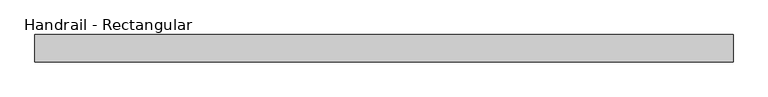
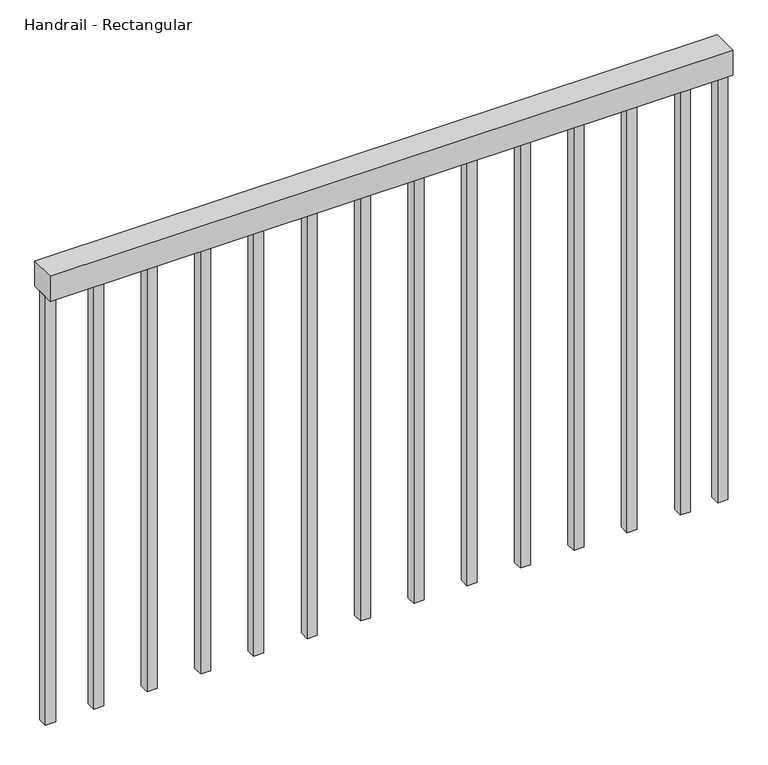
"""IFC4 building model written with IfcOpenShell, lengths in millimetres: railing geometry, Handrail - Rectangular."""

import ifcopenshell
import ifcopenshell.guid

model = None  # the IFC model being written
_history = None  # IfcOwnerHistory: only IFC2X3 demands one
_inside = {}  # id of a spatial element -> (the spatial element, [elements in it])
_under = {}  # id of a project, library or spatial element -> (it, [spatial elements below it])
_declared = {}  # id of a project -> (the project, [libraries it declares])
_typed = {}  # id of a type object -> (the type object, [elements of that type])
_made_of = {}  # id of a material, layer set ... -> (it, [elements and type objects made of it])


def new_model(schema):
    """Start an empty IFC model of exactly this schema.

    Asked for "IFC4X3", IfcOpenShell would pick the latest addendum, in which some entities
    have other attributes; the version numbers below select the first issue.
    IFC2X3 requires an IfcOwnerHistory on every rooted entity: one is made here for all.
    """
    global model, _history
    if schema == "IFC4X3":
        model = ifcopenshell.file(schema_version=(4, 3, 0, 0))
    else:
        model = ifcopenshell.file(schema=schema)
    _inside.clear()
    _under.clear()
    _declared.clear()
    _typed.clear()
    _made_of.clear()
    _history = None
    if model.schema == "IFC2X3":
        org = make("IfcOrganization", Name="unknown")
        user = make(
            "IfcPersonAndOrganization",
            ThePerson=make("IfcPerson", FamilyName="unknown"),
            TheOrganization=org,
        )
        app = make(
            "IfcApplication",
            ApplicationDeveloper=org,
            Version="unknown",
            ApplicationFullName="unknown",
            ApplicationIdentifier="unknown",
        )
        _history = make(
            "IfcOwnerHistory",
            OwningUser=user,
            OwningApplication=app,
            ChangeAction="ADDED",
            CreationDate=0,
        )
    return model


def make(cls, **values):
    """One entity of the class cls with the attributes given. An attribute that is None is left unset."""
    return model.create_entity(
        cls, **{name: value for name, value in values.items() if value is not None}
    )


def rooted(cls, **values):
    """An entity with a GlobalId (a new one), such as an element, a storey or a relation."""
    return make(cls, GlobalId=ifcopenshell.guid.new(), OwnerHistory=_history, **values)


def si_unit(unit_type, name, prefix=None):
    """IfcSIUnit, for example si_unit("LENGTHUNIT", "METRE", prefix="MILLI")."""
    return make("IfcSIUnit", UnitType=unit_type, Prefix=prefix, Name=name)


def assignment(units):
    """IfcUnitAssignment: the units of a project."""
    return None if units is None else make("IfcUnitAssignment", Units=units)


def point(xyz):
    """IfcCartesianPoint."""
    return None if xyz is None else make("IfcCartesianPoint", Coordinates=xyz)


def direction(xyz):
    """IfcDirection."""
    return None if xyz is None else make("IfcDirection", DirectionRatios=xyz)


def frame(location, z_axis=None, x_axis=None):
    """IfcAxis2Placement3D, a coordinate frame: its origin and axes. An axis left out is left unset."""
    return make(
        "IfcAxis2Placement3D",
        Location=point(location),
        Axis=direction(z_axis),
        RefDirection=direction(x_axis),
    )


def origin():
    """The frame at (0, 0, 0) with its axes left unset."""
    return frame((0.0, 0.0, 0.0))


def place(relative_to, where):
    """IfcLocalPlacement: puts the frame where relative to a parent placement (None: the world)."""
    return make(
        "IfcLocalPlacement", PlacementRelTo=relative_to, RelativePlacement=where
    )


def context(
    kind, dimensions, precision=None, world=None, true_north=None, identifier=None
):
    """IfcGeometricRepresentationContext, for example the 3D "Model" context."""
    return make(
        "IfcGeometricRepresentationContext",
        ContextIdentifier=identifier,
        ContextType=kind,
        CoordinateSpaceDimension=dimensions,
        Precision=precision,
        WorldCoordinateSystem=world,
        TrueNorth=true_north,
    )


def project(units=None, contexts=None):
    """IfcProject with its units and contexts."""
    return rooted(
        "IfcProject",
        Name="project",
        RepresentationContexts=contexts,
        UnitsInContext=assignment(units),
    )


def spatial(cls, under=None, at=None, **own):
    """A site, building, storey or space (cls), placed at a placement, below another one or the project."""
    s = rooted(cls, ObjectPlacement=at, **own)
    if under is not None:
        _under.setdefault(under.id(), (under, []))[1].append(s)
    return s


def polyline(points):
    """IfcPolyline through the points."""
    return make("IfcPolyline", Points=[point(p) for p in points])


def outline(outer, holes=None, kind="AREA"):
    """IfcArbitraryClosedProfileDef: a profile drawn as a closed curve; with holes, ...WithVoids."""
    if holes is None:
        return make("IfcArbitraryClosedProfileDef", ProfileType=kind, OuterCurve=outer)
    return make(
        "IfcArbitraryProfileDefWithVoids",
        ProfileType=kind,
        OuterCurve=outer,
        InnerCurves=holes,
    )


def extrude(swept, where, along, depth):
    """IfcExtrudedAreaSolid: the profile swept, set in the frame where, extruded along a direction by depth."""
    return make(
        "IfcExtrudedAreaSolid",
        SweptArea=swept,
        Position=where,
        ExtrudedDirection=direction(along),
        Depth=depth,
    )


def shape(context_of_items, identifier, shape_type, items):
    """IfcShapeRepresentation: the items that make up one representation, for example the "Body"."""
    return make(
        "IfcShapeRepresentation",
        ContextOfItems=context_of_items,
        RepresentationIdentifier=identifier,
        RepresentationType=shape_type,
        Items=items,
    )


def source(mapping_origin, context_of_items, identifier, shape_type, items):
    """IfcRepresentationMap: a shape defined once, which mapped items show again and again."""
    return make(
        "IfcRepresentationMap",
        MappingOrigin=mapping_origin,
        MappedRepresentation=shape(context_of_items, identifier, shape_type, items),
    )


def transform(
    local_origin,
    x_axis=None,
    y_axis=None,
    z_axis=None,
    scale=None,
    scale2=None,
    scale3=None,
    uniform=True,
):
    """IfcCartesianTransformationOperator3D, or its non-uniform kind. x_axis, y_axis, z_axis: its Axis1, 2, 3."""
    if uniform:
        return make(
            "IfcCartesianTransformationOperator3D",
            Axis1=direction(x_axis),
            Axis2=direction(y_axis),
            LocalOrigin=point(local_origin),
            Scale=scale,
            Axis3=direction(z_axis),
        )
    return make(
        "IfcCartesianTransformationOperator3DnonUniform",
        Axis1=direction(x_axis),
        Axis2=direction(y_axis),
        LocalOrigin=point(local_origin),
        Scale=scale,
        Axis3=direction(z_axis),
        Scale2=scale2,
        Scale3=scale3,
    )


def mapped(mapping_source, mapping_target):
    """IfcMappedItem: shows the shape of a source again, moved by a transform."""
    return make(
        "IfcMappedItem", MappingSource=mapping_source, MappingTarget=mapping_target
    )


def made_of(thing, what):
    """Note that an element or type object is made of a material, layer set ...; save() writes the relation."""
    if what is not None:
        _made_of.setdefault(what.id(), (what, []))[1].append(thing)
    return thing


def element(
    cls,
    number,
    at=None,
    inside=None,
    cuts=None,
    type_object=None,
    material=None,
    context=None,
    identifier="Body",
    shape_type=None,
    held_by="IfcProductDefinitionShape",
    body=None,
    shapes=None,
    **own,
):
    """One element of the class cls, such as IfcWall. Its Tag is "e" and its number.

    at: its placement. inside: the storey or other place that contains it. cuts: it is an
    opening in that element (IfcRelVoidsElement). A single representation is given by context,
    identifier, shape_type and body (its items); several are given by shapes. held_by: the class
    of the entity that holds the representations. save() writes the other relations.
    """
    e = rooted(cls, Tag="e%d" % number, ObjectPlacement=at, **own)
    if body is not None:
        shapes = [shape(context, identifier, shape_type, body)]
    if shapes is not None:
        e.Representation = make(held_by, Representations=shapes)
    if inside is not None:
        _inside.setdefault(inside.id(), (inside, []))[1].append(e)
    if cuts is not None:
        rooted(
            "IfcRelVoidsElement", RelatingBuildingElement=cuts, RelatedOpeningElement=e
        )
    if type_object is not None:
        _typed.setdefault(type_object.id(), (type_object, []))[1].append(e)
    return made_of(e, material)


def aggregate(whole, parts):
    """IfcRelAggregates: a whole, such as a stair, and the parts it consists of."""
    return rooted("IfcRelAggregates", RelatingObject=whole, RelatedObjects=parts)


def save(model, path):
    """Write the relations noted so far, then the file.

    IfcRelAggregates (storeys below a building ...), IfcRelContainedInSpatialStructure (elements
    in a storey), IfcRelDefinesByType, IfcRelAssociatesMaterial and IfcRelDeclares: one each for
    every whole, place, type object, material and project.
    """
    for whole, parts in _under.values():
        aggregate(whole, parts)
    for where, things in _inside.values():
        rooted(
            "IfcRelContainedInSpatialStructure",
            RelatedElements=things,
            RelatingStructure=where,
        )
    for kind, things in _typed.values():
        rooted("IfcRelDefinesByType", RelatedObjects=things, RelatingType=kind)
    for what, things in _made_of.values():
        rooted("IfcRelAssociatesMaterial", RelatedObjects=things, RelatingMaterial=what)
    for by, libraries in _declared.values():
        rooted("IfcRelDeclares", RelatingContext=by, RelatedDefinitions=libraries)
    model.write(path)


def handrail_rectangular_e98b01a6(model_context):
    return source(origin(), model_context, "Body", "SweptSolid", [
        extrude(outline(polyline([(614.7788909, 9945.0507146), (614.7788909, 9995.8507146), (1914.7788909, 9995.8507146), (1914.7788909, 9945.0507146), (614.7788909, 9945.0507146)])), frame((0.0, 0.0, 6654.4), z_axis=(0.0, 0.0, 1.0), x_axis=(1.0, 0.0, 0.0)), (0.0, 0.0, 1.0), 50.8),
        extrude(outline(polyline([(1824.4538909, 9960.9257146), (1824.4538909, 9979.9757146), (1843.5038909, 9979.9757146), (1843.5038909, 9960.9257146), (1824.4538909, 9960.9257146)])), frame((0.0, 0.0, 5790.8), z_axis=(0.0, 0.0, 1.0), x_axis=(1.0, 0.0, 0.0)), (0.0, 0.0, 1.0), 863.6),
        extrude(outline(polyline([(1722.8538909, 9960.9257146), (1722.8538909, 9979.9757146), (1741.9038909, 9979.9757146), (1741.9038909, 9960.9257146), (1722.8538909, 9960.9257146)])), frame((0.0, 0.0, 5790.8), z_axis=(0.0, 0.0, 1.0), x_axis=(1.0, 0.0, 0.0)), (0.0, 0.0, 1.0), 863.6),
        extrude(outline(polyline([(1621.2538909, 9960.9257146), (1621.2538909, 9979.9757146), (1640.3038909, 9979.9757146), (1640.3038909, 9960.9257146), (1621.2538909, 9960.9257146)])), frame((0.0, 0.0, 5790.8), z_axis=(0.0, 0.0, 1.0), x_axis=(1.0, 0.0, 0.0)), (0.0, 0.0, 1.0), 863.6),
        extrude(outline(polyline([(1519.6538909, 9960.9257146), (1519.6538909, 9979.9757146), (1538.7038909, 9979.9757146), (1538.7038909, 9960.9257146), (1519.6538909, 9960.9257146)])), frame((0.0, 0.0, 5790.8), z_axis=(0.0, 0.0, 1.0), x_axis=(1.0, 0.0, 0.0)), (0.0, 0.0, 1.0), 863.6),
        extrude(outline(polyline([(1418.0538909, 9960.9257146), (1418.0538909, 9979.9757146), (1437.1038909, 9979.9757146), (1437.1038909, 9960.9257146), (1418.0538909, 9960.9257146)])), frame((0.0, 0.0, 5790.8), z_axis=(0.0, 0.0, 1.0), x_axis=(1.0, 0.0, 0.0)), (0.0, 0.0, 1.0), 863.6),
        extrude(outline(polyline([(1316.4538909, 9960.9257146), (1316.4538909, 9979.9757146), (1335.5038909, 9979.9757146), (1335.5038909, 9960.9257146), (1316.4538909, 9960.9257146)])), frame((0.0, 0.0, 5790.8), z_axis=(0.0, 0.0, 1.0), x_axis=(1.0, 0.0, 0.0)), (0.0, 0.0, 1.0), 863.6),
        extrude(outline(polyline([(1214.8538909, 9960.9257146), (1214.8538909, 9979.9757146), (1233.9038909, 9979.9757146), (1233.9038909, 9960.9257146), (1214.8538909, 9960.9257146)])), frame((0.0, 0.0, 5790.8), z_axis=(0.0, 0.0, 1.0), x_axis=(1.0, 0.0, 0.0)), (0.0, 0.0, 1.0), 863.6),
        extrude(outline(polyline([(1113.2538909, 9960.9257146), (1113.2538909, 9979.9757146), (1132.3038909, 9979.9757146), (1132.3038909, 9960.9257146), (1113.2538909, 9960.9257146)])), frame((0.0, 0.0, 5790.8), z_axis=(0.0, 0.0, 1.0), x_axis=(1.0, 0.0, 0.0)), (0.0, 0.0, 1.0), 863.6),
        extrude(outline(polyline([(1011.6538909, 9960.9257146), (1011.6538909, 9979.9757146), (1030.7038909, 9979.9757146), (1030.7038909, 9960.9257146), (1011.6538909, 9960.9257146)])), frame((0.0, 0.0, 5790.8), z_axis=(0.0, 0.0, 1.0), x_axis=(1.0, 0.0, 0.0)), (0.0, 0.0, 1.0), 863.6),
        extrude(outline(polyline([(910.0538909, 9960.9257146), (910.0538909, 9979.9757146), (929.1038909, 9979.9757146), (929.1038909, 9960.9257146), (910.0538909, 9960.9257146)])), frame((0.0, 0.0, 5790.8), z_axis=(0.0, 0.0, 1.0), x_axis=(1.0, 0.0, 0.0)), (0.0, 0.0, 1.0), 863.6),
        extrude(outline(polyline([(808.4538909, 9960.9257146), (808.4538909, 9979.9757146), (827.5038909, 9979.9757146), (827.5038909, 9960.9257146), (808.4538909, 9960.9257146)])), frame((0.0, 0.0, 5790.8), z_axis=(0.0, 0.0, 1.0), x_axis=(1.0, 0.0, 0.0)), (0.0, 0.0, 1.0), 863.6),
        extrude(outline(polyline([(706.8538909, 9960.9257146), (706.8538909, 9979.9757146), (725.9038909, 9979.9757146), (725.9038909, 9960.9257146), (706.8538909, 9960.9257146)])), frame((0.0, 0.0, 5790.8), z_axis=(0.0, 0.0, 1.0), x_axis=(1.0, 0.0, 0.0)), (0.0, 0.0, 1.0), 863.6),
        extrude(outline(polyline([(1895.7288909, 9960.9257146), (1895.7288909, 9979.9757146), (1914.7788909, 9979.9757146), (1914.7788909, 9960.9257146), (1895.7288909, 9960.9257146)])), frame((0.0, 0.0, 5790.8), z_axis=(0.0, 0.0, 1.0), x_axis=(1.0, 0.0, 0.0)), (0.0, 0.0, 1.0), 863.6),
        extrude(outline(polyline([(614.7788909, 9960.9257146), (614.7788909, 9979.9757146), (633.8288909, 9979.9757146), (633.8288909, 9960.9257146), (614.7788909, 9960.9257146)])), frame((0.0, 0.0, 5790.8), z_axis=(0.0, 0.0, 1.0), x_axis=(1.0, 0.0, 0.0)), (0.0, 0.0, 1.0), 863.6),
    ])


if __name__ == "__main__":
    model = new_model("IFC4")
    model_context = context("Model", 3, world=origin())
    ifc_project = project(units=[si_unit("LENGTHUNIT", "METRE", prefix="MILLI")], contexts=[model_context])
    site = spatial("IfcSite", under=ifc_project)
    building = spatial("IfcBuilding", under=site)
    placement = place(None, origin())
    handrail_rectangular_shape = handrail_rectangular_e98b01a6(model_context)
    element("IfcRailing", 1, ObjectType="Handrail - Rectangular", at=placement, inside=building, context=model_context, shape_type="MappedRepresentation", body=[
        mapped(handrail_rectangular_shape, transform((0.0, 0.0, 0.0), x_axis=(1.0, 0.0, 0.0), y_axis=(0.0, 1.0, 0.0), z_axis=(0.0, 0.0, 1.0))),
    ])
    save(model, "model.ifc")
